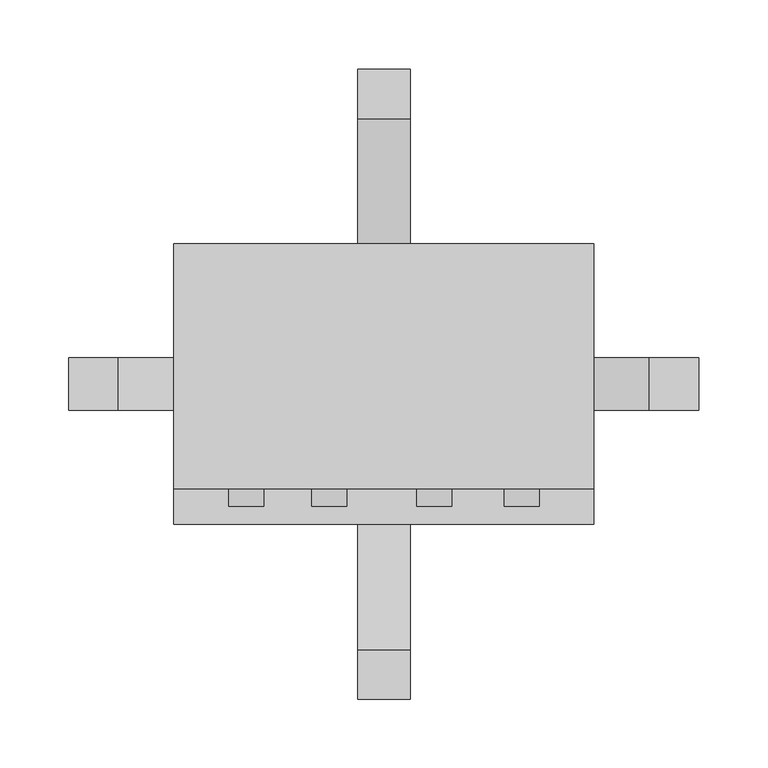
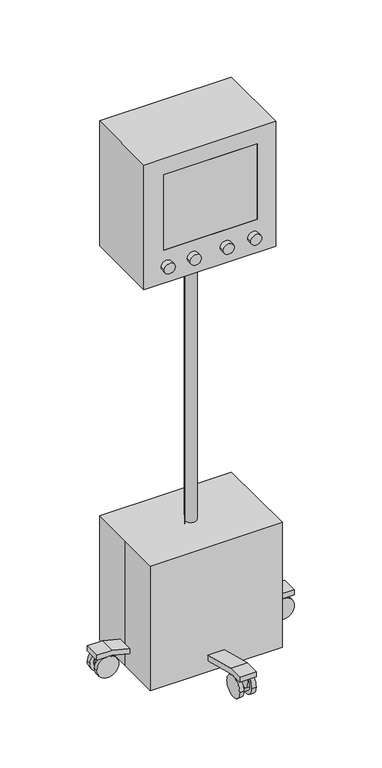
"""IFC4 building model written with IfcOpenShell, lengths in millimetres: proxy geometry, M7845 - Monitor, Physiological, Bedside, 4 Channel-mobile stand : M7845 - Monitor, Physiological, Bedside, 4 Channel-mobile stand."""

import ifcopenshell
import ifcopenshell.guid

model = None  # the IFC model being written
_history = None  # IfcOwnerHistory: only IFC2X3 demands one
_inside = {}  # id of a spatial element -> (the spatial element, [elements in it])
_under = {}  # id of a project, library or spatial element -> (it, [spatial elements below it])
_declared = {}  # id of a project -> (the project, [libraries it declares])
_typed = {}  # id of a type object -> (the type object, [elements of that type])
_made_of = {}  # id of a material, layer set ... -> (it, [elements and type objects made of it])


def new_model(schema):
    """Start an empty IFC model of exactly this schema.

    Asked for "IFC4X3", IfcOpenShell would pick the latest addendum, in which some entities
    have other attributes; the version numbers below select the first issue.
    IFC2X3 requires an IfcOwnerHistory on every rooted entity: one is made here for all.
    """
    global model, _history
    if schema == "IFC4X3":
        model = ifcopenshell.file(schema_version=(4, 3, 0, 0))
    else:
        model = ifcopenshell.file(schema=schema)
    _inside.clear()
    _under.clear()
    _declared.clear()
    _typed.clear()
    _made_of.clear()
    _history = None
    if model.schema == "IFC2X3":
        org = make("IfcOrganization", Name="unknown")
        user = make(
            "IfcPersonAndOrganization",
            ThePerson=make("IfcPerson", FamilyName="unknown"),
            TheOrganization=org,
        )
        app = make(
            "IfcApplication",
            ApplicationDeveloper=org,
            Version="unknown",
            ApplicationFullName="unknown",
            ApplicationIdentifier="unknown",
        )
        _history = make(
            "IfcOwnerHistory",
            OwningUser=user,
            OwningApplication=app,
            ChangeAction="ADDED",
            CreationDate=0,
        )
    return model


def make(cls, **values):
    """One entity of the class cls with the attributes given. An attribute that is None is left unset."""
    return model.create_entity(
        cls, **{name: value for name, value in values.items() if value is not None}
    )


def rooted(cls, **values):
    """An entity with a GlobalId (a new one), such as an element, a storey or a relation."""
    return make(cls, GlobalId=ifcopenshell.guid.new(), OwnerHistory=_history, **values)


def si_unit(unit_type, name, prefix=None):
    """IfcSIUnit, for example si_unit("LENGTHUNIT", "METRE", prefix="MILLI")."""
    return make("IfcSIUnit", UnitType=unit_type, Prefix=prefix, Name=name)


def assignment(units):
    """IfcUnitAssignment: the units of a project."""
    return None if units is None else make("IfcUnitAssignment", Units=units)


def point(xyz):
    """IfcCartesianPoint."""
    return None if xyz is None else make("IfcCartesianPoint", Coordinates=xyz)


def direction(xyz):
    """IfcDirection."""
    return None if xyz is None else make("IfcDirection", DirectionRatios=xyz)


def frame(location, z_axis=None, x_axis=None):
    """IfcAxis2Placement3D, a coordinate frame: its origin and axes. An axis left out is left unset."""
    return make(
        "IfcAxis2Placement3D",
        Location=point(location),
        Axis=direction(z_axis),
        RefDirection=direction(x_axis),
    )


def frame_2d(location, x_axis=None):
    """IfcAxis2Placement2D, a coordinate frame in the plane: its origin and x axis."""
    return make(
        "IfcAxis2Placement2D", Location=point(location), RefDirection=direction(x_axis)
    )


def origin():
    """The frame at (0, 0, 0) with its axes left unset."""
    return frame((0.0, 0.0, 0.0))


def origin_with_axes():
    """The frame at (0, 0, 0) with the z axis (0, 0, 1) and the x axis (1, 0, 0) written out."""
    return frame((0.0, 0.0, 0.0), z_axis=(0.0, 0.0, 1.0), x_axis=(1.0, 0.0, 0.0))


def place(relative_to, where):
    """IfcLocalPlacement: puts the frame where relative to a parent placement (None: the world)."""
    return make(
        "IfcLocalPlacement", PlacementRelTo=relative_to, RelativePlacement=where
    )


def context(
    kind, dimensions, precision=None, world=None, true_north=None, identifier=None
):
    """IfcGeometricRepresentationContext, for example the 3D "Model" context."""
    return make(
        "IfcGeometricRepresentationContext",
        ContextIdentifier=identifier,
        ContextType=kind,
        CoordinateSpaceDimension=dimensions,
        Precision=precision,
        WorldCoordinateSystem=world,
        TrueNorth=true_north,
    )


def project(units=None, contexts=None):
    """IfcProject with its units and contexts."""
    return rooted(
        "IfcProject",
        Name="project",
        RepresentationContexts=contexts,
        UnitsInContext=assignment(units),
    )


def spatial(cls, under=None, at=None, **own):
    """A site, building, storey or space (cls), placed at a placement, below another one or the project."""
    s = rooted(cls, ObjectPlacement=at, **own)
    if under is not None:
        _under.setdefault(under.id(), (under, []))[1].append(s)
    return s


def polyline(points):
    """IfcPolyline through the points."""
    return make("IfcPolyline", Points=[point(p) for p in points])


def circle_curve(where, radius):
    """IfcCircle in the frame where."""
    return make("IfcCircle", Position=where, Radius=radius)


def trimmed(basis, trim1, trim2, sense, master):
    """IfcTrimmedCurve: the piece of a basis curve between two trims."""
    return make(
        "IfcTrimmedCurve",
        BasisCurve=basis,
        Trim1=trim1,
        Trim2=trim2,
        SenseAgreement=sense,
        MasterRepresentation=master,
    )


def segment(curve, same_sense, transition):
    """IfcCompositeCurveSegment."""
    return make(
        "IfcCompositeCurveSegment",
        Transition=transition,
        SameSense=same_sense,
        ParentCurve=curve,
    )


def composite_curve(segments, self_intersect=None):
    """IfcCompositeCurve: segments joined end to end."""
    return make("IfcCompositeCurve", Segments=segments, SelfIntersect=self_intersect)


def outline(outer, holes=None, kind="AREA"):
    """IfcArbitraryClosedProfileDef: a profile drawn as a closed curve; with holes, ...WithVoids."""
    if holes is None:
        return make("IfcArbitraryClosedProfileDef", ProfileType=kind, OuterCurve=outer)
    return make(
        "IfcArbitraryProfileDefWithVoids",
        ProfileType=kind,
        OuterCurve=outer,
        InnerCurves=holes,
    )


def extrude(swept, where, along, depth):
    """IfcExtrudedAreaSolid: the profile swept, set in the frame where, extruded along a direction by depth."""
    return make(
        "IfcExtrudedAreaSolid",
        SweptArea=swept,
        Position=where,
        ExtrudedDirection=direction(along),
        Depth=depth,
    )


def faces_of(points, faces, orient=None, outer=None):
    """IfcFace entities. A face is a list of loops; a loop is a list of indices into points, from 0.

    orient and outer hold one flag for each loop. By default every Orientation is true, the
    first loop of a face is its IfcFaceOuterBound and the others are IfcFaceBound.
    """
    made = []
    for i, loops in enumerate(faces):
        bounds = []
        for j, loop in enumerate(loops):
            is_outer = j == 0 if outer is None else outer[i][j]
            bounds.append(
                make(
                    "IfcFaceOuterBound" if is_outer else "IfcFaceBound",
                    Bound=make("IfcPolyLoop", Polygon=[points[k] for k in loop]),
                    Orientation=True if orient is None else orient[i][j],
                )
            )
        made.append(make("IfcFace", Bounds=bounds))
    return made


def faceted_brep(points, faces, orient=None, outer=None, voids=None):
    """IfcFacetedBrep: a solid bounded by flat faces; with voids (closed shells), ...WithVoids."""
    shared = [point(p) for p in points]
    hull = make("IfcClosedShell", CfsFaces=faces_of(shared, faces, orient, outer))
    if voids is None:
        return make("IfcFacetedBrep", Outer=hull)
    return make(
        "IfcFacetedBrepWithVoids",
        Outer=hull,
        Voids=[
            make(cls, CfsFaces=faces_of(shared, fs, o, b)) for cls, fs, o, b in voids
        ],
    )


def shape(context_of_items, identifier, shape_type, items):
    """IfcShapeRepresentation: the items that make up one representation, for example the "Body"."""
    return make(
        "IfcShapeRepresentation",
        ContextOfItems=context_of_items,
        RepresentationIdentifier=identifier,
        RepresentationType=shape_type,
        Items=items,
    )


def source(mapping_origin, context_of_items, identifier, shape_type, items):
    """IfcRepresentationMap: a shape defined once, which mapped items show again and again."""
    return make(
        "IfcRepresentationMap",
        MappingOrigin=mapping_origin,
        MappedRepresentation=shape(context_of_items, identifier, shape_type, items),
    )


def transform(
    local_origin,
    x_axis=None,
    y_axis=None,
    z_axis=None,
    scale=None,
    scale2=None,
    scale3=None,
    uniform=True,
):
    """IfcCartesianTransformationOperator3D, or its non-uniform kind. x_axis, y_axis, z_axis: its Axis1, 2, 3."""
    if uniform:
        return make(
            "IfcCartesianTransformationOperator3D",
            Axis1=direction(x_axis),
            Axis2=direction(y_axis),
            LocalOrigin=point(local_origin),
            Scale=scale,
            Axis3=direction(z_axis),
        )
    return make(
        "IfcCartesianTransformationOperator3DnonUniform",
        Axis1=direction(x_axis),
        Axis2=direction(y_axis),
        LocalOrigin=point(local_origin),
        Scale=scale,
        Axis3=direction(z_axis),
        Scale2=scale2,
        Scale3=scale3,
    )


def mapped(mapping_source, mapping_target):
    """IfcMappedItem: shows the shape of a source again, moved by a transform."""
    return make(
        "IfcMappedItem", MappingSource=mapping_source, MappingTarget=mapping_target
    )


def made_of(thing, what):
    """Note that an element or type object is made of a material, layer set ...; save() writes the relation."""
    if what is not None:
        _made_of.setdefault(what.id(), (what, []))[1].append(thing)
    return thing


def element(
    cls,
    number,
    at=None,
    inside=None,
    cuts=None,
    type_object=None,
    material=None,
    context=None,
    identifier="Body",
    shape_type=None,
    held_by="IfcProductDefinitionShape",
    body=None,
    shapes=None,
    **own,
):
    """One element of the class cls, such as IfcWall. Its Tag is "e" and its number.

    at: its placement. inside: the storey or other place that contains it. cuts: it is an
    opening in that element (IfcRelVoidsElement). A single representation is given by context,
    identifier, shape_type and body (its items); several are given by shapes. held_by: the class
    of the entity that holds the representations. save() writes the other relations.
    """
    e = rooted(cls, Tag="e%d" % number, ObjectPlacement=at, **own)
    if body is not None:
        shapes = [shape(context, identifier, shape_type, body)]
    if shapes is not None:
        e.Representation = make(held_by, Representations=shapes)
    if inside is not None:
        _inside.setdefault(inside.id(), (inside, []))[1].append(e)
    if cuts is not None:
        rooted(
            "IfcRelVoidsElement", RelatingBuildingElement=cuts, RelatedOpeningElement=e
        )
    if type_object is not None:
        _typed.setdefault(type_object.id(), (type_object, []))[1].append(e)
    return made_of(e, material)


def aggregate(whole, parts):
    """IfcRelAggregates: a whole, such as a stair, and the parts it consists of."""
    return rooted("IfcRelAggregates", RelatingObject=whole, RelatedObjects=parts)


def save(model, path):
    """Write the relations noted so far, then the file.

    IfcRelAggregates (storeys below a building ...), IfcRelContainedInSpatialStructure (elements
    in a storey), IfcRelDefinesByType, IfcRelAssociatesMaterial and IfcRelDeclares: one each for
    every whole, place, type object, material and project.
    """
    for whole, parts in _under.values():
        aggregate(whole, parts)
    for where, things in _inside.values():
        rooted(
            "IfcRelContainedInSpatialStructure",
            RelatedElements=things,
            RelatingStructure=where,
        )
    for kind, things in _typed.values():
        rooted("IfcRelDefinesByType", RelatedObjects=things, RelatingType=kind)
    for what, things in _made_of.values():
        rooted("IfcRelAssociatesMaterial", RelatedObjects=things, RelatingMaterial=what)
    for by, libraries in _declared.values():
        rooted("IfcRelDeclares", RelatingContext=by, RelatedDefinitions=libraries)
    model.write(path)


def specialty_equipment_808a7331(model_context):
    return source(origin(), model_context, "Body", "SolidModel", [
        extrude(outline(composite_curve([segment(trimmed(circle_curve(frame_2d((203.0677083, 25.4)), 25.4), [point((228.4677083, 25.4))], [point((177.6677083, 25.4))], False, "CARTESIAN"), True, "CONTINUOUS"), segment(trimmed(circle_curve(frame_2d((203.0677083, 25.4)), 25.4), [point((177.6677083, 25.4))], [point((228.4677083, 25.4))], False, "CARTESIAN"), True, "CONTINUOUS")], self_intersect=False)), frame((9.4354799, 0.0, 0.0), z_axis=(1.0, 0.0, 0.0), x_axis=(0.0, 1.0, 0.0)), (0.0, 0.0, 1.0), 9.525),
        extrude(outline(composite_curve([segment(trimmed(circle_curve(frame_2d((203.0677083, 25.4)), 25.4), [point((177.6677083, 25.4))], [point((228.4677083, 25.4))], False, "CARTESIAN"), True, "CONTINUOUS"), segment(trimmed(circle_curve(frame_2d((203.0677083, 25.4)), 25.4), [point((228.4677083, 25.4))], [point((177.6677083, 25.4))], False, "CARTESIAN"), True, "CONTINUOUS")], self_intersect=False)), frame((-19.1395201, 0.0, 0.0), z_axis=(1.0, 0.0, 0.0), x_axis=(0.0, 1.0, 0.0)), (0.0, 0.0, 1.0), 9.525),
        extrude(outline(composite_curve([segment(trimmed(circle_curve(frame_2d((25.4, 203.1766257)), 25.4), [point((25.4, 177.7766257))], [point((25.4, 228.5766257))], False, "CARTESIAN"), True, "CONTINUOUS"), segment(trimmed(circle_curve(frame_2d((25.4, 203.1766257)), 25.4), [point((25.4, 228.5766257))], [point((25.4, 177.7766257))], False, "CARTESIAN"), True, "CONTINUOUS")], self_intersect=False)), frame((0.0, -19.05, 0.0), z_axis=(0.0, 1.0, 0.0), x_axis=(0.0, 0.0, 1.0)), (0.0, 0.0, 1.0), 9.525),
        extrude(outline(composite_curve([segment(trimmed(circle_curve(frame_2d((25.4, 203.1766257)), 25.4), [point((25.4, 177.7766257))], [point((25.4, 228.5766257))], False, "CARTESIAN"), True, "CONTINUOUS"), segment(trimmed(circle_curve(frame_2d((25.4, 203.1766257)), 25.4), [point((25.4, 228.5766257))], [point((25.4, 177.7766257))], False, "CARTESIAN"), True, "CONTINUOUS")], self_intersect=False)), frame((0.0, 9.525, 0.0), z_axis=(0.0, 1.0, 0.0), x_axis=(0.0, 0.0, 1.0)), (0.0, 0.0, 1.0), 9.525),
        extrude(outline(composite_curve([segment(trimmed(circle_curve(frame_2d((25.4, -203.1572284)), 25.4), [point((25.4, -228.5572284))], [point((25.4, -177.7572284))], False, "CARTESIAN"), True, "CONTINUOUS"), segment(trimmed(circle_curve(frame_2d((25.4, -203.1572284)), 25.4), [point((25.4, -177.7572284))], [point((25.4, -228.5572284))], False, "CARTESIAN"), True, "CONTINUOUS")], self_intersect=False)), frame((0.0, 9.525, 0.0), z_axis=(0.0, 1.0, 0.0), x_axis=(0.0, 0.0, 1.0)), (0.0, 0.0, 1.0), 9.525),
        extrude(outline(composite_curve([segment(trimmed(circle_curve(frame_2d((25.4, -203.1572284)), 25.4), [point((25.4, -177.7572284))], [point((25.4, -228.5572284))], False, "CARTESIAN"), True, "CONTINUOUS"), segment(trimmed(circle_curve(frame_2d((25.4, -203.1572284)), 25.4), [point((25.4, -228.5572284))], [point((25.4, -177.7572284))], False, "CARTESIAN"), True, "CONTINUOUS")], self_intersect=False)), frame((0.0, -19.05, 0.0), z_axis=(0.0, 1.0, 0.0), x_axis=(0.0, 0.0, 1.0)), (0.0, 0.0, 1.0), 9.525),
        extrude(outline(composite_curve([segment(trimmed(circle_curve(frame_2d((-203.2165365, 25.4)), 25.4), [point((-177.8165365, 25.4))], [point((-228.6165365, 25.4))], False, "CARTESIAN"), True, "CONTINUOUS"), segment(trimmed(circle_curve(frame_2d((-203.2165365, 25.4)), 25.4), [point((-228.6165365, 25.4))], [point((-177.8165365, 25.4))], False, "CARTESIAN"), True, "CONTINUOUS")], self_intersect=False)), frame((-19.1395201, 0.0, 0.0), z_axis=(1.0, 0.0, 0.0), x_axis=(0.0, 1.0, 0.0)), (0.0, 0.0, 1.0), 9.525),
        extrude(outline(composite_curve([segment(trimmed(circle_curve(frame_2d((-203.2165365, 25.4)), 25.4), [point((-177.8165365, 25.4))], [point((-228.6165365, 25.4))], False, "CARTESIAN"), True, "CONTINUOUS"), segment(trimmed(circle_curve(frame_2d((-203.2165365, 25.4)), 25.4), [point((-228.6165365, 25.4))], [point((-177.8165365, 25.4))], False, "CARTESIAN"), True, "CONTINUOUS")], self_intersect=False)), frame((9.4354799, 0.0, 0.0), z_axis=(1.0, 0.0, 0.0), x_axis=(0.0, 1.0, 0.0)), (0.0, 0.0, 1.0), 9.525),
        extrude(outline(composite_curve([segment(trimmed(circle_curve(frame_2d((-0.0895201, 211.534375)), 8.4666667), [point((-8.5561868, 211.534375))], [point((8.3771466, 211.534375))], False, "CARTESIAN"), True, "CONTINUOUS"), segment(trimmed(circle_curve(frame_2d((-0.0895201, 211.534375)), 8.4666667), [point((8.3771466, 211.534375))], [point((-8.5561868, 211.534375))], False, "CARTESIAN"), True, "CONTINUOUS")], self_intersect=False)), frame((0.0, 0.0, 25.4), z_axis=(0.0, 0.0, 1.0), x_axis=(1.0, 0.0, 0.0)), (0.0, 0.0, 1.0), 25.4),
        extrude(outline(composite_curve([segment(trimmed(circle_curve(frame_2d((203.0677083, 25.4)), 16.9333333), [point((186.134375, 25.4))], [point((220.0010417, 25.4))], False, "CARTESIAN"), True, "CONTINUOUS"), segment(trimmed(circle_curve(frame_2d((203.0677083, 25.4)), 16.9333333), [point((220.0010417, 25.4))], [point((186.134375, 25.4))], False, "CARTESIAN"), True, "CONTINUOUS")], self_intersect=False)), frame((-9.6145201, 0.0, 0.0), z_axis=(1.0, 0.0, 0.0), x_axis=(0.0, 1.0, 0.0)), (0.0, 0.0, 1.0), 19.05),
        extrude(outline(composite_curve([segment(trimmed(circle_curve(frame_2d((211.6432924, 0.0)), 8.4666667), [point((211.6432924, 8.4666667))], [point((211.6432924, -8.4666667))], False, "CARTESIAN"), True, "CONTINUOUS"), segment(trimmed(circle_curve(frame_2d((211.6432924, 0.0)), 8.4666667), [point((211.6432924, -8.4666667))], [point((211.6432924, 8.4666667))], False, "CARTESIAN"), True, "CONTINUOUS")], self_intersect=False)), frame((0.0, 0.0, 25.4), z_axis=(0.0, 0.0, 1.0), x_axis=(1.0, 0.0, 0.0)), (0.0, 0.0, 1.0), 25.4),
        extrude(outline(composite_curve([segment(trimmed(circle_curve(frame_2d((25.4, 203.1766257)), 16.9333333), [point((25.4, 186.2432924))], [point((25.4, 220.1099591))], False, "CARTESIAN"), True, "CONTINUOUS"), segment(trimmed(circle_curve(frame_2d((25.4, 203.1766257)), 16.9333333), [point((25.4, 220.1099591))], [point((25.4, 186.2432924))], False, "CARTESIAN"), True, "CONTINUOUS")], self_intersect=False)), frame((0.0, -9.525, 0.0), z_axis=(0.0, 1.0, 0.0), x_axis=(0.0, 0.0, 1.0)), (0.0, 0.0, 1.0), 19.05),
        extrude(outline(composite_curve([segment(trimmed(circle_curve(frame_2d((-211.6238951, 0.0)), 8.4666667), [point((-211.6238951, -8.4666667))], [point((-211.6238951, 8.4666667))], False, "CARTESIAN"), True, "CONTINUOUS"), segment(trimmed(circle_curve(frame_2d((-211.6238951, 0.0)), 8.4666667), [point((-211.6238951, 8.4666667))], [point((-211.6238951, -8.4666667))], False, "CARTESIAN"), True, "CONTINUOUS")], self_intersect=False)), frame((0.0, 0.0, 25.4), z_axis=(0.0, 0.0, 1.0), x_axis=(1.0, 0.0, 0.0)), (0.0, 0.0, 1.0), 25.4),
        extrude(outline(composite_curve([segment(trimmed(circle_curve(frame_2d((25.4, -203.1572284)), 16.9333333), [point((25.4, -186.2238951))], [point((25.4, -220.0905618))], False, "CARTESIAN"), True, "CONTINUOUS"), segment(trimmed(circle_curve(frame_2d((25.4, -203.1572284)), 16.9333333), [point((25.4, -220.0905618))], [point((25.4, -186.2238951))], False, "CARTESIAN"), True, "CONTINUOUS")], self_intersect=False)), frame((0.0, -9.525, 0.0), z_axis=(0.0, 1.0, 0.0), x_axis=(0.0, 0.0, 1.0)), (0.0, 0.0, 1.0), 19.05),
        extrude(outline(composite_curve([segment(trimmed(circle_curve(frame_2d((-0.0895201, -211.6832031)), 8.4666667), [point((8.3771466, -211.6832031))], [point((-8.5561868, -211.6832031))], False, "CARTESIAN"), True, "CONTINUOUS"), segment(trimmed(circle_curve(frame_2d((-0.0895201, -211.6832031)), 8.4666667), [point((-8.5561868, -211.6832031))], [point((8.3771466, -211.6832031))], False, "CARTESIAN"), True, "CONTINUOUS")], self_intersect=False)), frame((0.0, 0.0, 25.4), z_axis=(0.0, 0.0, 1.0), x_axis=(1.0, 0.0, 0.0)), (0.0, 0.0, 1.0), 25.4),
        extrude(outline(composite_curve([segment(trimmed(circle_curve(frame_2d((-203.2165365, 25.4)), 16.9333333), [point((-186.2832031, 25.4))], [point((-220.1498698, 25.4))], False, "CARTESIAN"), True, "CONTINUOUS"), segment(trimmed(circle_curve(frame_2d((-203.2165365, 25.4)), 16.9333333), [point((-220.1498698, 25.4))], [point((-186.2832031, 25.4))], False, "CARTESIAN"), True, "CONTINUOUS")], self_intersect=False)), frame((-9.6145201, 0.0, 0.0), z_axis=(1.0, 0.0, 0.0), x_axis=(0.0, 1.0, 0.0)), (0.0, 0.0, 1.0), 19.05),
        extrude(outline(polyline([(-228.6, 63.5), (-192.6166667, 63.5), (-44.45, 25.4), (44.45, 25.4), (192.6166667, 63.5), (228.6, 63.5), (228.6, 50.8), (193.8216772, 50.8), (45.6550105, 12.7), (-45.6550105, 12.7), (-193.8216772, 50.8), (-228.6, 50.8), (-228.6, 63.5)])), frame((-19.1395201, 0.0, 0.0), z_axis=(1.0, 0.0, 0.0), x_axis=(0.0, 1.0, 0.0)), (0.0, 0.0, 1.0), 38.1),
        extrude(outline(composite_curve([segment(trimmed(circle_curve(frame_2d((-0.0895201, 0.0)), 12.7), [point((-12.7895201, 0.0))], [point((12.6104799, 0.0))], False, "CARTESIAN"), True, "CONTINUOUS"), segment(trimmed(circle_curve(frame_2d((-0.0895201, 0.0)), 12.7), [point((12.6104799, 0.0))], [point((-12.7895201, 0.0))], False, "CARTESIAN"), True, "CONTINUOUS")], self_intersect=False)), frame((0.0, 0.0, 12.7), z_axis=(0.0, 0.0, 1.0), x_axis=(1.0, 0.0, 0.0)), (0.0, 0.0, 1.0), 952.5),
        extrude(outline(polyline([(63.5, -228.6895201), (50.8, -228.6895201), (50.8, -193.9111973), (12.7, -45.7445306), (12.7, 45.5654904), (50.8, 193.7321571), (50.8, 228.5104799), (63.5, 228.5104799), (63.5, 192.5271466), (25.4, 44.3604799), (25.4, -44.5395201), (63.5, -192.7061868), (63.5, -228.6895201)])), frame((0.0, -19.05, 0.0), z_axis=(0.0, 1.0, 0.0), x_axis=(0.0, 0.0, 1.0)), (0.0, 0.0, 1.0), 38.1),
        extrude(outline(composite_curve([segment(trimmed(circle_curve(frame_2d((1006.3587525, 100.0366492)), 12.7), [point((1006.3587525, 112.7366492))], [point((1006.3587525, 87.3366492))], False, "CARTESIAN"), True, "CONTINUOUS"), segment(trimmed(circle_curve(frame_2d((1006.3587525, 100.0366492)), 12.7), [point((1006.3587525, 87.3366492))], [point((1006.3587525, 112.7366492))], False, "CARTESIAN"), True, "CONTINUOUS")], self_intersect=False)), frame((0.0, -88.9, 0.0), z_axis=(0.0, 1.0, 0.0), x_axis=(0.0, 0.0, 1.0)), (0.0, 0.0, 1.0), 12.7),
        extrude(outline(composite_curve([segment(trimmed(circle_curve(frame_2d((1006.3587525, -39.7116492)), 12.7), [point((1006.3587525, -52.4116492))], [point((1006.3587525, -27.0116492))], False, "CARTESIAN"), True, "CONTINUOUS"), segment(trimmed(circle_curve(frame_2d((1006.3587525, -39.7116492)), 12.7), [point((1006.3587525, -27.0116492))], [point((1006.3587525, -52.4116492))], False, "CARTESIAN"), True, "CONTINUOUS")], self_intersect=False)), frame((0.0, -88.9, 0.0), z_axis=(0.0, 1.0, 0.0), x_axis=(0.0, 0.0, 1.0)), (0.0, 0.0, 1.0), 12.7),
        extrude(outline(composite_curve([segment(trimmed(circle_curve(frame_2d((1006.3587525, -100.0366492)), 12.7), [point((1006.3587525, -112.7366492))], [point((1006.3587525, -87.3366492))], False, "CARTESIAN"), True, "CONTINUOUS"), segment(trimmed(circle_curve(frame_2d((1006.3587525, -100.0366492)), 12.7), [point((1006.3587525, -87.3366492))], [point((1006.3587525, -112.7366492))], False, "CARTESIAN"), True, "CONTINUOUS")], self_intersect=False)), frame((0.0, -88.9, 0.0), z_axis=(0.0, 1.0, 0.0), x_axis=(0.0, 0.0, 1.0)), (0.0, 0.0, 1.0), 12.7),
        extrude(outline(composite_curve([segment(trimmed(circle_curve(frame_2d((1006.3587525, 36.4883508)), 12.7), [point((1006.3587525, 23.7883508))], [point((1006.3587525, 49.1883508))], False, "CARTESIAN"), True, "CONTINUOUS"), segment(trimmed(circle_curve(frame_2d((1006.3587525, 36.4883508)), 12.7), [point((1006.3587525, 49.1883508))], [point((1006.3587525, 23.7883508))], False, "CARTESIAN"), True, "CONTINUOUS")], self_intersect=False)), frame((0.0, -88.9, 0.0), z_axis=(0.0, 1.0, 0.0), x_axis=(0.0, 0.0, 1.0)), (0.0, 0.0, 1.0), 12.7),
        extrude(outline(polyline([(109.187649, -76.2), (-106.712351, -76.2), (-106.712351, -69.85), (109.187649, -69.85), (109.187649, -76.2)])), frame((0.0, 0.0, 1046.2028485), z_axis=(0.0, 0.0, 1.0), x_axis=(1.0, 0.0, 0.0)), (0.0, 0.0, 1.0), 184.15),
        faceted_brep([(152.4, -76.2, 1270.0), (-152.4, -76.2, 1270.0), (-152.4, -76.2, 965.2), (152.4, -76.2, 965.2), (-106.712351, -76.2, 1230.3528485), (109.187649, -76.2, 1230.3528485), (109.187649, -76.2, 1046.2028485), (-106.712351, -76.2, 1046.2028485), (152.4, 101.6, 1270.0), (152.4, 101.6, 965.2), (-152.4, 101.6, 965.2), (-152.4, 101.6, 1270.0), (109.187649, -63.5, 1230.3528485), (-106.712351, -63.5, 1230.3528485), (-106.712351, -63.5, 1046.2028485), (109.187649, -63.5, 1046.2028485)], [[[0, 1, 2, 3], [4, 5, 6, 7]], [[8, 9, 10, 11]], [[1, 0, 8, 11]], [[2, 1, 11, 10]], [[3, 2, 10, 9]], [[0, 3, 9, 8]], [[12, 13, 14, 15]], [[13, 12, 5, 4]], [[14, 13, 4, 7]], [[15, 14, 7, 6]], [[12, 15, 6, 5]]]),
        extrude(outline(polyline([(-152.4, 101.6), (152.4, 101.6), (152.4, -101.6), (-152.4, -101.6), (-152.4, 0.0), (-152.4, 101.6)])), origin_with_axes(), (0.0, 0.0, 1.0), 304.8),
    ])


if __name__ == "__main__":
    model = new_model("IFC4")
    model_context = context("Model", 3, world=origin())
    ifc_project = project(units=[si_unit("LENGTHUNIT", "METRE", prefix="MILLI")], contexts=[model_context])
    site = spatial("IfcSite", under=ifc_project)
    building = spatial("IfcBuilding", under=site)
    placement = place(None, origin())
    specialty_equipment_shape = specialty_equipment_808a7331(model_context)
    element("IfcBuildingElementProxy", 1, Name="M7845 - Monitor, Physiological, Bedside, 4 Channel-mobile stand : M7845 - Monitor, Physiological, Bedside, 4 Channel-mobile stand", ObjectType="M7845 - Monitor, Physiological, Bedside, 4 Channel-mobile stand : M7845 - Monitor, Physiological, Bedside, 4 Channel-mobile stand", at=placement, inside=building, context=model_context, shape_type="MappedRepresentation", body=[
        mapped(specialty_equipment_shape, transform((0.0, 0.0, 0.0), x_axis=(1.0, 0.0, 0.0), y_axis=(0.0, 1.0, 0.0), z_axis=(0.0, 0.0, 1.0))),
    ])
    save(model, "model.ifc")

# Revit data of these elements
# Project information
#   Room Abbreviation = "VEX02"
#   Room Description = "Procedure, Veterinary (VEX02)"
#   Sheets - Total = "5"
#   Project Issue Date = "Issue Date"
#   Project Status = "Project Status"
#   Client Name = "Owner"
#   Project Address = "Enter address here"
#   Project Name = "Project Name"
#   Project Number = "Project Number"
#   Publication Date = "30-Jan-15"
# Type "M7845 - Monitor, Physiological, Bedside, 4 Channel-mobile stand : M7845 - Monitor, Physiological, Bedside, 4 Channel-mobile stand"
#   Watts2 = "0"
#   Watts1 = "360"
#   Unit_Issue = "EA"
#   UTIL_6_Misc = "D"
#   UTIL_5_NonMedGas = "-"
#   UTIL_4_MiscGas = "-"
#   UTIL_3_MedGas = "-"
#   UTIL_2_Elec = "A"
#   UTIL_1_WaterDrain = "-"
#   Nomenclature = "Monitor, Physiological, Bedside, 4 Channel"
#   NSN = "6515"
#   Location [instance default] = ""
#   JSN = "M7845"
#   Fund_Source_VA = "-"
#   Fund_Source_Navy = "-"
#   Fund_Source_Army = "-"
#   Fund_Source_AF = "-"
#   ELEC_Volts2 = "0"
#   ELEC_Volts1 = "120"
#   ELEC_Phase2 = "0"
#   ELEC_Phase1 = "1"
#   ELEC_HertzSwitch = "0"
#   ELEC_HertzDependent = "-1"
#   ELEC_Hertz = "60"
#   ELEC_Amps2 = "0"
#   ELEC_Amps1 = "3"
#   DetailDescription = "4 channel bedside physiological monitor. The unit consist of a four-channel non-fade monochrome display monitor, an alarm system and printer-recording capabilities. The monitor has color coded controls and automatic calibration. The unit displays up to four waveforms simultaneously. The parameters to be monitored are user selectable. The monitor may be connected to a central monitoring station. The unit monitors patients in most acute care areas, step-down units, procedure rooms and emergency rooms."
#   CAT_VA = "C"
#   CAT_Navy = "C"
#   CAT_IHS = "-"
#   CAT_Army = "C"
#   CAT_AF = "C"
#   BTUperhour = "0"
#   Weight_IP = 12
#   DIM_Width_IP = 1' - 0"
#   DIM_Height_IP = 1' - 0"
#   DIM_Depth_IP = 0' - 8"
#   finish [instance default] = none
# Element 1 (IfcBuildingElementProxy, "M7845 - Monitor, Physiological, Bedside, 4 Channel-mobile stand : M7845 - Monitor, Physiological, Bedside, 4 Channel-mobile stand")
#   Materials on its faces: "EquipSpace", "Glass"
# Materials
#   "EquipSpace": class "Unassigned", colour RGB 221 217 195, transparency 0.5
#   "Glass": class "Glass", colour RGB 0 128 192, transparency 0.75
